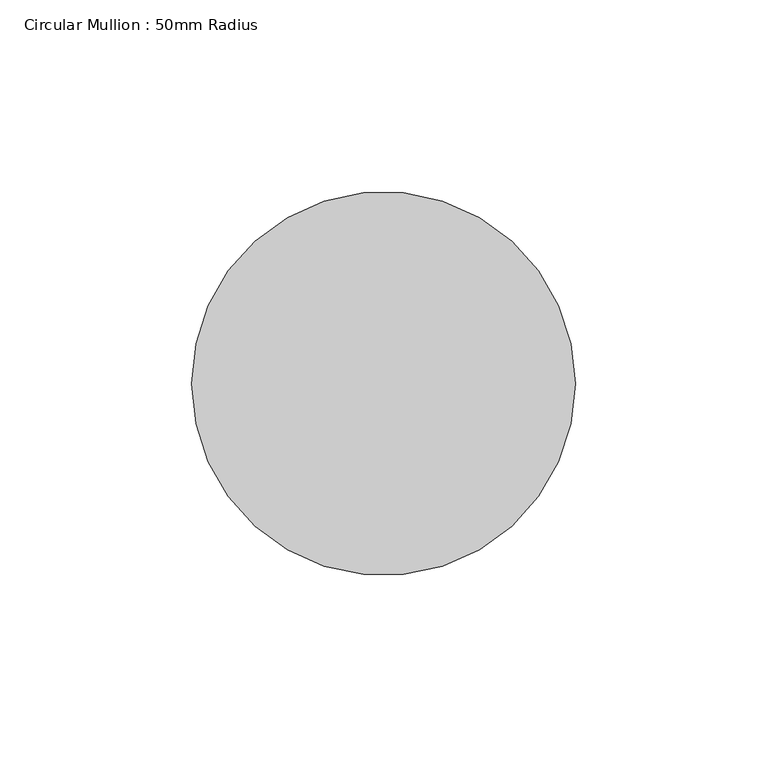
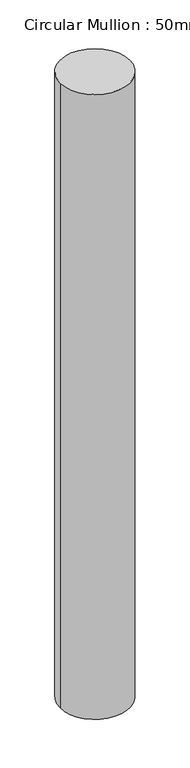
"""IFC4 building model written with IfcOpenShell, lengths in millimetres: member geometry, Circular Mullion : 50mm Radius."""

from ifc_helpers import new_model, si_unit, point, frame, origin, origin_2d, place, context, project, spatial, circle_curve, trimmed, segment, composite_curve, outline, extrude, source, transform, mapped, element, save


def circular_mullion_50mm_radius_c824747d(model_context):
    return source(origin(), model_context, "Body", "SweptSolid", [
        extrude(outline(composite_curve([segment(trimmed(circle_curve(origin_2d(), 50.0), [point((50.0, 0.0))], [point((-50.0, 0.0))], False, "CARTESIAN"), True, "CONTINUOUS"), segment(trimmed(circle_curve(origin_2d(), 50.0), [point((-50.0, 0.0))], [point((50.0, 0.0))], False, "CARTESIAN"), True, "CONTINUOUS")], self_intersect=False)), frame((0.0, 0.0, -951.3613403), z_axis=(0.0, 0.0, 1.0), x_axis=(1.0, 0.0, 0.0)), (0.0, 0.0, 1.0), 951.3613403),
    ])


if __name__ == "__main__":
    model = new_model("IFC4")
    model_context = context("Model", 3, world=origin())
    ifc_project = project(units=[si_unit("LENGTHUNIT", "METRE", prefix="MILLI")], contexts=[model_context])
    site = spatial("IfcSite", under=ifc_project)
    building = spatial("IfcBuilding", under=site)
    placement = place(None, origin())
    circular_mullion_50mm_radius_shape = circular_mullion_50mm_radius_c824747d(model_context)
    element("IfcMember", 1, ObjectType="Circular Mullion : 50mm Radius", at=placement, inside=building, context=model_context, shape_type="MappedRepresentation", body=[
        mapped(circular_mullion_50mm_radius_shape, transform((0.0, 0.0, 0.0), x_axis=(1.0, 0.0, 0.0), y_axis=(0.0, 1.0, 0.0), z_axis=(0.0, 0.0, 1.0))),
    ])
    save(model, "model.ifc")

# Revit data of these elements
# Type "Circular Mullion : 50mm Radius"
#   built-in parameter 1007350 = 0.164042 (stored number, unit not read)
# Element 1 (IfcMember, "Circular Mullion : 50mm Radius")
#   Materials on its faces: "Aluminium"
# Materials
#   "Aluminium": class "Metal", colour RGB 247 247 247, transparency 0, Description = "Aluminium 6061", Cost = 0
